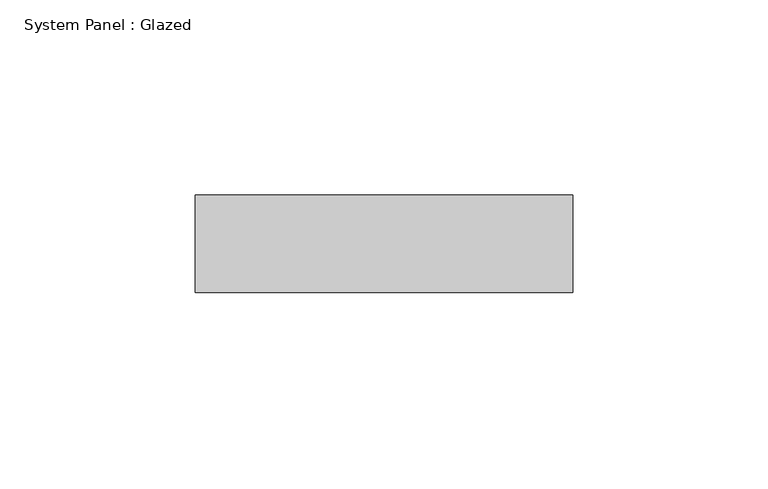
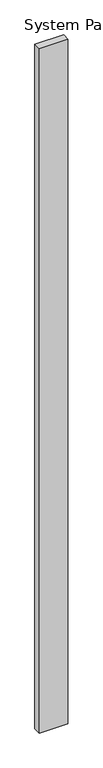
"""IFC4 building model written with IfcOpenShell, lengths in millimetres: plate geometry, System Panel : Glazed."""

from ifc_helpers import new_model, si_unit, origin, origin_with_axes, place, context, project, spatial, polyline, outline, extrude, source, transform, mapped, element, save


def system_panel_glazed_a471ea82(model_context):
    return source(origin(), model_context, "Body", "SweptSolid", [
        extrude(outline(polyline([(48.4090908, 24.5), (-48.4090908, 24.5), (-48.4090908, 49.5), (48.4090908, 49.5), (48.4090908, 24.5)])), origin_with_axes(), (0.0, 0.0, 1.0), 2435.0),
    ])


if __name__ == "__main__":
    model = new_model("IFC4")
    model_context = context("Model", 3, world=origin())
    ifc_project = project(units=[si_unit("LENGTHUNIT", "METRE", prefix="MILLI")], contexts=[model_context])
    site = spatial("IfcSite", under=ifc_project)
    building = spatial("IfcBuilding", under=site)
    placement = place(None, origin())
    system_panel_glazed_shape = system_panel_glazed_a471ea82(model_context)
    element("IfcPlate", 1, ObjectType="System Panel : Glazed", at=placement, inside=building, context=model_context, shape_type="MappedRepresentation", body=[
        mapped(system_panel_glazed_shape, transform((0.0, 0.0, 0.0), x_axis=(1.0, 0.0, 0.0), y_axis=(0.0, 1.0, 0.0), z_axis=(0.0, 0.0, 1.0))),
    ])
    save(model, "model.ifc")

# Revit data of these elements
# Element 1 (IfcPlate, "System Panel : Glazed")
#   Materials on its faces: "Glass"
# Materials
#   "Glass": class "Glass", colour RGB 218 227 224, transparency 0.85, Description = "Soda Lime Glass", Cost = 0
